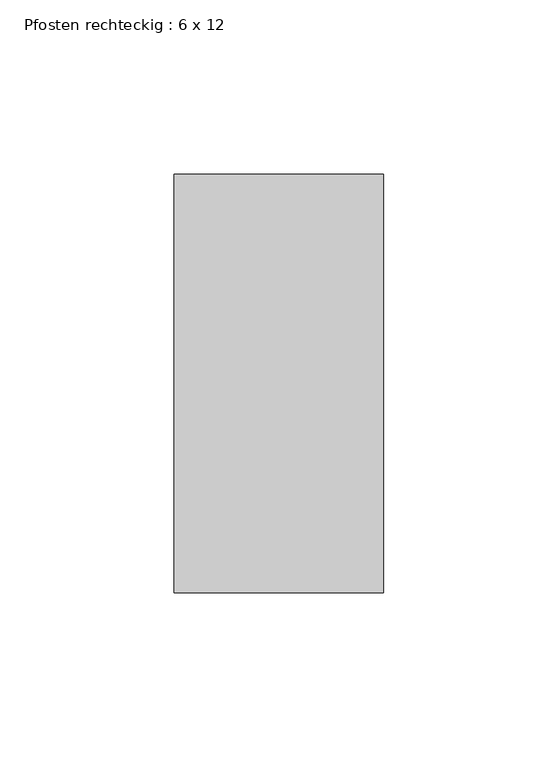
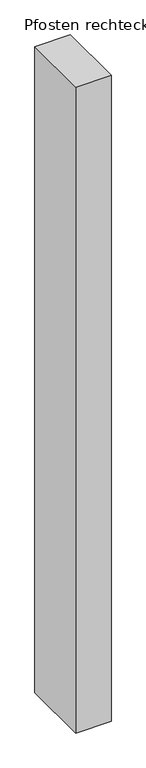
"""IFC4 building model written with IfcOpenShell, lengths in millimetres: member geometry, Pfosten rechteckig : 6 x 12."""

from ifc_helpers import new_model, si_unit, frame, origin, place, context, project, spatial, polyline, outline, extrude, source, transform, mapped, element, save


def pfosten_rechteckig_6_x_12_9384716b(model_context):
    return source(origin(), model_context, "Body", "SweptSolid", [
        extrude(outline(polyline([(0.0, 60.0), (0.0, -60.0), (-60.0, -60.0), (-60.0, 60.0), (0.0, 60.0)])), frame((0.0, 0.0, -1160.0000003), z_axis=(0.0, 0.0, 1.0), x_axis=(1.0, 0.0, 0.0)), (0.0, 0.0, 1.0), 1160.0000003),
    ])


if __name__ == "__main__":
    model = new_model("IFC4")
    model_context = context("Model", 3, world=origin())
    ifc_project = project(units=[si_unit("LENGTHUNIT", "METRE", prefix="MILLI")], contexts=[model_context])
    site = spatial("IfcSite", under=ifc_project)
    building = spatial("IfcBuilding", under=site)
    placement = place(None, origin())
    pfosten_rechteckig_6_x_12_shape = pfosten_rechteckig_6_x_12_9384716b(model_context)
    element("IfcMember", 1, ObjectType="Pfosten rechteckig : 6 x 12", at=placement, inside=building, context=model_context, shape_type="MappedRepresentation", body=[
        mapped(pfosten_rechteckig_6_x_12_shape, transform((0.0, 0.0, 0.0), x_axis=(1.0, 0.0, 0.0), y_axis=(0.0, 1.0, 0.0), z_axis=(0.0, 0.0, 1.0))),
    ])
    save(model, "model.ifc")

# Revit data of these elements
# Type "Pfosten rechteckig : 6 x 12"
#   built-in parameter 1007304 = 0.393701 (stored number, unit not read)
#   built-in parameter 1007301 = 0.0984252 (stored number, unit not read)
#   built-in parameter 1007300 = 0.0984252 (stored number, unit not read)
# Element 1 (IfcMember, "Pfosten rechteckig : 6 x 12")
#   Materials on its faces: "Metall - verzinkt"
# Materials
#   "Metall - verzinkt": class "Allgemeines", colour RGB 200 200 200, transparency 0, Cost = 0
